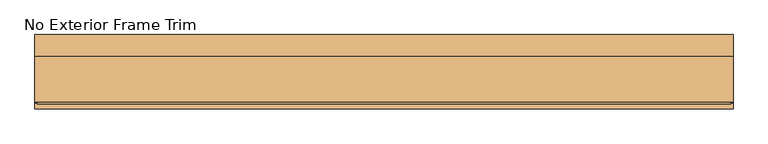
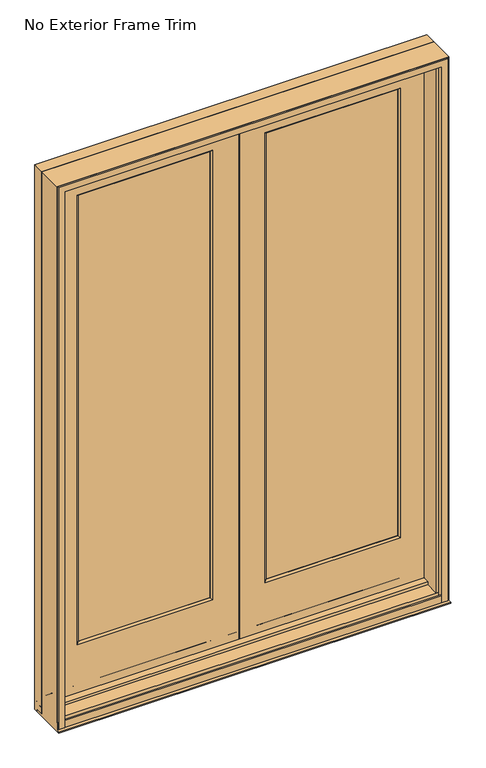
"""IFC4 building model written with IfcOpenShell, lengths in millimetres: door geometry, Door-In_Swing-Milgard-Essence-2_Panel : No Exterior Frame Trim."""

from ifc_helpers import new_model, si_unit, frame, origin, place, context, project, spatial, polyline, outline, extrude, faceted_brep, source, transform, mapped, element, save


def no_exterior_frame_trim_898b5155(model_context):
    return source(origin(), model_context, "Body", "SolidModel", [
        extrude(outline(polyline([(591.4684989, -34.925), (54.2422052, -34.925), (54.2422052, -9.525), (591.4684989, -9.525), (591.4684989, -34.925)])), frame((0.0, 0.0, 245.0465023), z_axis=(0.0, 0.0, 1.0), x_axis=(1.0, 0.0, 0.0)), (0.0, 0.0, 1.0), 1856.965426),
        faceted_brep([(-22.501829, -7.1755004, 39.0524923), (-39.8139839, -7.1755004, 39.0524923), (-39.8139839, 1.1430002, 39.0524923), (685.524688, 1.1430002, 39.0524923), (685.524688, -7.1755004, 39.0524923), (668.2125331, -7.1755004, 39.0524923), (665.7443122, -10.2234994, 39.0524923), (597.9581931, -10.2234994, 39.0524923), (597.9581931, -8.4581998, 39.0524923), (583.7647037, -8.4581998, 39.0524923), (582.2411552, -9.525, 39.0524923), (578.7581009, -9.525, 39.0524923), (578.7581009, -7.642861, 39.0524923), (579.0279319, -7.1755004, 39.0524923), (66.6827722, -7.1755004, 39.0524923), (66.9526032, -7.642861, 39.0524923), (66.9526032, -9.525, 39.0524923), (63.4695489, -9.525, 39.0524923), (61.9460004, -8.4581998, 39.0524923), (47.7525111, -8.4581998, 39.0524923), (47.7525111, -10.2234994, 39.0524923), (-20.0336081, -10.2234994, 39.0524923), (-22.501829, -7.1755004, 2178.7559624), (-22.501829, -7.1755004, 257.4235308), (-22.1233678, -7.642861, 257.6933617), (-20.5992417, -9.525, 257.6933617), (-20.5992417, -9.525, 254.2103075), (-21.4631194, -8.4581998, 252.686759), (-21.4631194, -8.4581998, 238.4932696), (-20.0336081, -10.2234994, 238.4932696), (-20.0336081, -10.2234994, 2176.2877415), (-20.0336081, -10.2234994, 58.8285873), (-22.501829, -7.1755004, 56.3603664), (47.7525111, -10.2234994, 58.8285873), (597.9581931, -10.2234994, 58.8285873), (665.7443122, -10.2234994, 58.8285873), (685.524688, -10.2234994, 58.8285873), (685.524688, -10.2234994, 238.4932696), (665.7443122, -10.2234994, 238.4932696), (665.7443122, -10.2234994, 2176.2877415), (-39.8139839, -10.2234994, 238.4932696), (-39.8139839, -10.2234994, 58.8285873), (47.7525111, -10.2234994, 2108.5016224), (597.9581931, -10.2234994, 2108.5016224), (597.9581931, -10.2234994, 238.4932696), (47.7525111, -10.2234994, 238.4932696), (47.7525111, -8.4581998, 238.4932696), (47.7525111, -8.4581998, 252.686759), (47.7525111, -9.525, 254.2103075), (47.7525111, -9.525, 257.6933617), (47.7525111, -8.4581998, 257.6933617), (47.7525111, -8.4581998, 2108.5016224), (47.7525111, -8.4581998, 57.3990759), (597.9581931, -8.4581998, 57.3990759), (583.7647037, -8.4581998, 57.3990759), (61.9460004, -8.4581998, 238.4932696), (61.9460004, -8.4581998, 252.686759), (61.9460004, -8.4581998, 257.6933617), (61.9460004, -8.4581998, 2094.3081331), (583.7647037, -8.4581998, 2094.3081331), (583.7647037, -8.4581998, 257.6933617), (597.9581931, -8.4581998, 257.6933617), (597.9581931, -8.4581998, 2108.5016224), (597.9581931, -8.4581998, 252.686759), (583.7647037, -8.4581998, 252.686759), (583.7647037, -8.4581998, 238.4932696), (597.9581931, -8.4581998, 238.4932696), (61.9460004, -8.4581998, 57.3990759), (63.4695489, -9.525, 238.4932696), (63.4695489, -9.525, 254.2103075), (63.4695489, -9.525, 257.6933617), (63.4695489, -9.525, 2092.7845845), (63.4695489, -9.525, 58.2629537), (582.2411552, -9.525, 58.2629537), (578.7581009, -9.525, 58.2629537), (66.9526032, -9.525, 238.4932696), (66.9526032, -9.525, 254.2103075), (578.7581009, -9.525, 254.2103075), (578.7581009, -9.525, 238.4932696), (582.2411552, -9.525, 238.4932696), (582.2411552, -9.525, 254.2103075), (597.9581931, -9.525, 254.2103075), (597.9581931, -9.525, 257.6933617), (582.2411552, -9.525, 257.6933617), (582.2411552, -9.525, 2092.7845845), (66.9526032, -9.525, 2089.3015303), (578.7581009, -9.525, 2089.3015303), (578.7581009, -9.525, 257.6933617), (66.9526032, -9.525, 257.6933617), (685.524688, -9.525, 257.6933617), (666.3099458, -9.525, 257.6933617), (666.3099458, -9.525, 254.2103075), (685.524688, -9.525, 254.2103075), (66.9526032, -9.525, 58.2629537), (-39.8139839, -9.525, 254.2103075), (-39.8139839, -9.525, 257.6933617), (66.9526032, -8.4581998, 238.4932696), (66.9526032, -8.4581998, 252.686759), (66.9526032, -7.642861, 257.6933617), (66.9526032, -7.642861, 2089.3015303), (66.9526032, -7.642861, 56.7388275), (66.6827722, -7.1755004, 56.3603664), (62.3383529, 0.3492502, 253.0791115), (62.3383529, 0.3492502, 2093.9157805), (597.9581931, 0.3492502, 2108.5016224), (597.9581931, 0.3492502, 238.4932696), (47.7525111, 0.3492502, 238.4932696), (47.7525111, 0.3492502, 2108.5016224), (583.3723512, 0.3492502, 253.0791115), (583.3723512, 0.3492502, 2093.9157805), (47.7525111, 1.1430002, 238.4932696), (47.7525111, 1.1430002, 2108.5016224), (-39.8139839, 1.1430002, 2196.0681173), (685.524688, 1.1430002, 2196.0681173), (597.9581931, 1.1430002, 2108.5016224), (597.9581931, 1.1430002, 238.4932696), (-39.8139839, -7.1755004, 56.3603664), (-39.8139839, -8.4581998, 238.4932696), (-39.8139839, -8.4581998, 252.686759), (-39.8139839, -7.642861, 257.6933617), (-39.8139839, -7.1755004, 257.4235308), (-39.8139839, -7.1755004, 2196.0681173), (685.524688, -7.1755004, 56.3603664), (668.2125331, -7.1755004, 56.3603664), (668.2125331, -7.1755004, 2178.7559624), (668.2125331, -7.1755004, 257.4235308), (685.524688, -7.1755004, 257.4235308), (685.524688, -7.1755004, 2196.0681173), (578.7581009, -7.642861, 2089.3015303), (667.1738236, -8.4581998, 238.4932696), (667.1738236, -8.4581998, 252.686759), (667.8340719, -7.642861, 257.6933617), (578.7581009, -7.642861, 56.7388275), (578.7581009, -8.4581998, 252.686759), (578.7581009, -8.4581998, 238.4932696), (578.7581009, -7.642861, 257.6933617), (579.0279319, -7.1755004, 56.3603664), (685.524688, -7.642861, 257.6933617), (685.524688, -8.4581998, 252.686759), (685.524688, -8.4581998, 238.4932696)], [[[0, 1, 2, 3, 4, 5, 6, 7, 8, 9, 10, 11, 12, 13, 14, 15, 16, 17, 18, 19, 20, 21]], [[22, 23, 24, 25, 26, 27, 28, 29, 30]], [[21, 31, 32, 0]], [[20, 33, 34, 7, 6, 35, 36, 37, 38, 39, 30, 29, 40, 41, 31, 21], [42, 43, 44, 45]], [[42, 45, 46, 47, 48, 49, 50, 51]], [[19, 52, 33, 20]], [[8, 53, 54, 9]], [[46, 55, 56, 47]], [[51, 50, 57, 58, 59, 60, 61, 62]], [[63, 64, 65, 66]], [[18, 67, 52, 19]], [[55, 68, 69, 56]], [[58, 57, 70, 71]], [[17, 72, 67, 18]], [[10, 73, 74, 11]], [[71, 70, 49, 48, 69, 68, 75, 76, 77, 78, 79, 80, 81, 82, 83, 84], [85, 86, 87, 88]], [[89, 90, 91, 92]], [[16, 93, 72, 17]], [[94, 26, 25, 95]], [[75, 96, 97, 76]], [[85, 88, 98, 99]], [[15, 100, 93, 16]], [[14, 101, 100, 15]], [[99, 98, 102, 103]], [[104, 105, 106, 107], [103, 102, 108, 109]], [[106, 110, 111, 107]], [[2, 112, 113, 3], [114, 111, 110, 115]], [[1, 116, 41, 40, 117, 118, 94, 95, 119, 120, 121, 112, 2]], [[0, 32, 116, 1]], [[4, 122, 123, 5]], [[121, 120, 23, 22, 124, 125, 126, 127]], [[30, 39, 124, 22]], [[42, 51, 62, 43]], [[58, 71, 84, 59]], [[85, 99, 128, 86]], [[103, 109, 128, 99]], [[107, 111, 114, 104]], [[112, 121, 127, 113]], [[39, 38, 129, 130, 91, 90, 131, 125, 124]], [[5, 123, 35, 6]], [[62, 61, 82, 81, 63, 66, 44, 43]], [[7, 34, 53, 8]], [[84, 83, 60, 59]], [[9, 54, 73, 10]], [[79, 65, 64, 80]], [[11, 74, 132, 12]], [[77, 133, 134, 78]], [[128, 135, 87, 86]], [[109, 108, 135, 128]], [[12, 132, 136, 13]], [[114, 115, 105, 104]], [[127, 126, 137, 89, 92, 138, 139, 37, 36, 122, 4, 3, 113]], [[105, 115, 110, 106]], [[102, 98, 135, 108]], [[126, 125, 131, 137]], [[119, 24, 23, 120]], [[70, 57, 50, 49]], [[95, 25, 24, 119]], [[82, 61, 60, 83]], [[87, 135, 98, 88]], [[137, 131, 90, 89]], [[48, 47, 56, 69]], [[76, 97, 133, 77]], [[80, 64, 63, 81]], [[92, 91, 130, 138]], [[118, 27, 26, 94]], [[97, 96, 134, 133]], [[138, 130, 129, 139]], [[117, 28, 27, 118]], [[40, 29, 28, 117]], [[44, 66, 65, 79, 78, 134, 96, 75, 68, 55, 46, 45]], [[139, 129, 38, 37]], [[33, 52, 67, 72, 93, 100, 101, 136, 132, 74, 73, 54, 53, 34]], [[116, 32, 31, 41]], [[36, 35, 123, 122]], [[13, 136, 101, 14]]]),
        faceted_brep([(-39.8139839, -43.3070016, 39.0524923), (-39.8139839, -43.3070016, 2196.0681173), (-39.8139839, -7.1755004, 2196.0681173), (-39.8139839, -7.1755004, 39.0524923), (685.524688, -7.1755004, 39.0524923), (685.524688, -7.1755004, 2196.0681173), (685.524688, -43.3070016, 2196.0681173), (685.524688, -43.3070016, 39.0524923), (66.7863819, -36.1729967, 257.5271404), (59.6523769, -43.3070016, 250.3931355), (586.0583272, -43.3070016, 250.3931355), (578.9243222, -36.1729967, 257.5271404), (59.6523769, -43.3070016, 2096.6017565), (586.0583272, -43.3070016, 2096.6017565), (669.6356705, -7.1755004, 55.4786786), (669.6356705, -7.1755004, 2180.1790999), (-23.9249664, -7.1755004, 2180.1790999), (-23.9249664, -7.1755004, 55.4786786), (-20.8769674, -10.2234994, 57.9468995), (666.5876715, -10.2234994, 57.9468995), (666.5876715, -10.2234994, 2177.1311009), (-20.8769674, -10.2234994, 2177.1311009), (594.7531877, -10.2234994, 241.698275), (594.7531877, -10.2234994, 2105.296617), (50.9575164, -10.2234994, 2105.296617), (50.9575164, -10.2234994, 241.698275), (50.9575164, -12.6518919, 241.698275), (594.7531877, -12.6518919, 241.698275), (49.0643221, -12.6518919, 2107.1898114), (49.0643221, -12.6518919, 239.8050807), (596.646382, -12.6518919, 239.8050807), (596.646382, -12.6518919, 2107.1898114), (50.9575164, -12.6518919, 2105.296617), (594.7531877, -12.6518919, 2105.296617), (47.7525111, -16.6892311, 238.4932696), (597.9581931, -16.6892311, 238.4932696), (47.7525111, -35.6615995, 238.4932696), (64.012343, -35.6615995, 238.4932696), (64.7489425, -34.925, 238.4932696), (66.7863819, -34.925, 238.4932696), (66.7863819, -35.6615995, 238.4932696), (578.9243222, -35.6615995, 238.4932696), (578.9243222, -34.925, 238.4932696), (580.9617616, -34.925, 238.4932696), (581.6983611, -35.6615995, 238.4932696), (597.9581931, -35.6615995, 238.4932696), (581.6983611, -35.6615995, 254.7531016), (597.9581931, -35.6615995, 254.7531016), (66.7863819, -35.6615995, 254.7531016), (578.9243222, -35.6615995, 254.7531016), (47.7525111, -35.6615995, 254.7531016), (64.012343, -35.6615995, 254.7531016), (47.7525111, -34.925, 255.4897011), (64.7489425, -34.925, 255.4897011), (66.7863819, -34.925, 255.4897011), (578.9243222, -34.925, 255.4897011), (580.9617616, -34.925, 255.4897011), (597.9581931, -34.925, 255.4897011), (47.7525111, -34.925, 257.5271404), (64.7489425, -34.925, 257.5271404), (64.7489425, -34.925, 2091.505191), (580.9617616, -34.925, 2091.505191), (580.9617616, -34.925, 257.5271404), (597.9581931, -34.925, 257.5271404), (578.9243222, -34.925, 257.5271404), (578.9243222, -34.925, 2089.4677516), (66.7863819, -34.925, 2089.4677516), (66.7863819, -34.925, 257.5271404), (581.6983611, -35.6615995, 257.5271404), (597.9581931, -35.6615995, 257.5271404), (47.7525111, -35.6615995, 257.5271404), (64.012343, -35.6615995, 257.5271404), (66.7863819, -36.1729967, 2089.4677516), (64.012343, -35.6615995, 2092.2417904), (47.7525111, -35.6615995, 2108.5016224), (597.9581931, -35.6615995, 2108.5016224), (581.6983611, -35.6615995, 2092.2417904), (47.7525111, -16.6892311, 2108.5016224), (578.9243222, -36.1729967, 2089.4677516), (597.9581931, -16.6892311, 2108.5016224)], [[[0, 1, 2, 3]], [[4, 5, 6, 7]], [[8, 9, 10, 11]], [[0, 7, 6, 1], [9, 12, 13, 10]], [[4, 7, 0, 3]], [[2, 5, 4, 3], [14, 15, 16, 17]], [[17, 18, 19, 14]], [[20, 19, 18, 21], [22, 23, 24, 25]], [[25, 26, 27, 22]], [[28, 29, 30, 31], [26, 32, 33, 27]], [[29, 34, 35, 30]], [[34, 36, 37, 38, 39, 40, 41, 42, 43, 44, 45, 35]], [[44, 46, 47, 45]], [[40, 48, 49, 41]], [[36, 50, 51, 37]], [[50, 52, 53, 51]], [[48, 54, 55, 49]], [[46, 56, 57, 47]], [[52, 58, 59, 60, 61, 62, 63, 57, 56, 43, 42, 55, 54, 39, 38, 53], [64, 65, 66, 67]], [[11, 64, 67, 8]], [[62, 68, 69, 63]], [[58, 70, 71, 59]], [[12, 9, 8, 72]], [[54, 48, 40, 39]], [[72, 8, 67, 66]], [[38, 37, 51, 53]], [[60, 59, 71, 73]], [[73, 71, 70, 74, 75, 69, 68, 76]], [[74, 70, 58, 52, 50, 36, 34, 77]], [[77, 34, 29, 28]], [[32, 26, 25, 24]], [[18, 17, 16, 21]], [[12, 72, 78, 13]], [[66, 65, 78, 72]], [[60, 73, 76, 61]], [[74, 77, 79, 75]], [[28, 31, 79, 77]], [[32, 24, 23, 33]], [[21, 16, 15, 20]], [[6, 5, 2, 1]], [[78, 11, 10, 13]], [[42, 41, 49, 55]], [[65, 64, 11, 78]], [[56, 46, 44, 43]], [[76, 68, 62, 61]], [[79, 35, 45, 47, 57, 63, 69, 75]], [[30, 35, 79, 31]], [[23, 22, 27, 33]], [[15, 14, 19, 20]]]),
        extrude(outline(polyline([(-675.754549, -34.925), (-675.754549, -9.525), (-138.5282552, -9.525), (-138.5282552, -34.925), (-675.754549, -34.925)])), frame((0.0, 0.0, 245.0465023), z_axis=(0.0, 0.0, 1.0), x_axis=(1.0, 0.0, 0.0)), (0.0, 0.0, 1.0), 1856.965426),
        faceted_brep([(-61.784221, -7.1755004, 39.0524923), (-64.252442, -10.2234994, 39.0524923), (-132.0385611, -10.2234994, 39.0524923), (-132.0385611, -8.4581998, 39.0524923), (-146.2320504, -8.4581998, 39.0524923), (-147.755599, -9.525, 39.0524923), (-151.2386532, -9.525, 39.0524923), (-151.2386532, -7.642861, 39.0524923), (-150.9688223, -7.1755004, 39.0524923), (-663.3139819, -7.1755004, 39.0524923), (-663.044151, -7.642861, 39.0524923), (-663.044151, -9.525, 39.0524923), (-666.5272052, -9.525, 39.0524923), (-668.0507537, -8.4581998, 39.0524923), (-682.2442431, -8.4581998, 39.0524923), (-682.2442431, -10.2234994, 39.0524923), (-750.0303622, -10.2234994, 39.0524923), (-752.4985831, -7.1755004, 39.0524923), (-769.810738, -7.1755004, 39.0524923), (-769.810738, 1.1430002, 39.0524923), (-44.4720661, 1.1430002, 39.0524923), (-44.4720661, -7.1755004, 39.0524923), (-61.784221, -7.1755004, 56.3603664), (-64.252442, -10.2234994, 58.8285873), (-61.784221, -7.1755004, 2178.7559624), (-64.252442, -10.2234994, 2176.2877415), (-64.252442, -10.2234994, 238.4932696), (-62.8229306, -8.4581998, 238.4932696), (-62.8229306, -8.4581998, 252.686759), (-63.6868083, -9.525, 254.2103075), (-63.6868083, -9.525, 257.6933617), (-62.1626822, -7.642861, 257.6933617), (-61.784221, -7.1755004, 257.4235308), (-44.4720661, -10.2234994, 58.8285873), (-44.4720661, -10.2234994, 238.4932696), (-750.0303622, -10.2234994, 2176.2877415), (-750.0303622, -10.2234994, 238.4932696), (-769.810738, -10.2234994, 238.4932696), (-769.810738, -10.2234994, 58.8285873), (-750.0303622, -10.2234994, 58.8285873), (-682.2442431, -10.2234994, 58.8285873), (-132.0385611, -10.2234994, 58.8285873), (-132.0385611, -10.2234994, 2108.5016224), (-132.0385611, -10.2234994, 238.4932696), (-682.2442431, -10.2234994, 238.4932696), (-682.2442431, -10.2234994, 2108.5016224), (-132.0385611, -8.4581998, 57.3990759), (-132.0385611, -8.4581998, 2108.5016224), (-132.0385611, -8.4581998, 257.6933617), (-132.0385611, -9.525, 257.6933617), (-132.0385611, -9.525, 254.2103075), (-132.0385611, -8.4581998, 252.686759), (-132.0385611, -8.4581998, 238.4932696), (-668.0507537, -8.4581998, 57.3990759), (-682.2442431, -8.4581998, 57.3990759), (-146.2320504, -8.4581998, 57.3990759), (-682.2442431, -8.4581998, 2108.5016224), (-682.2442431, -8.4581998, 257.6933617), (-668.0507537, -8.4581998, 257.6933617), (-668.0507537, -8.4581998, 2094.3081331), (-146.2320504, -8.4581998, 2094.3081331), (-146.2320504, -8.4581998, 257.6933617), (-146.2320504, -8.4581998, 252.686759), (-146.2320504, -8.4581998, 238.4932696), (-682.2442431, -8.4581998, 252.686759), (-682.2442431, -8.4581998, 238.4932696), (-668.0507537, -8.4581998, 238.4932696), (-668.0507537, -8.4581998, 252.686759), (-147.755599, -9.525, 58.2629537), (-147.755599, -9.525, 2092.7845845), (-147.755599, -9.525, 257.6933617), (-147.755599, -9.525, 254.2103075), (-147.755599, -9.525, 238.4932696), (-663.044151, -9.525, 58.2629537), (-666.5272052, -9.525, 58.2629537), (-151.2386532, -9.525, 58.2629537), (-666.5272052, -9.525, 2092.7845845), (-666.5272052, -9.525, 257.6933617), (-682.2442431, -9.525, 257.6933617), (-682.2442431, -9.525, 254.2103075), (-666.5272052, -9.525, 254.2103075), (-666.5272052, -9.525, 238.4932696), (-663.044151, -9.525, 238.4932696), (-663.044151, -9.525, 254.2103075), (-151.2386532, -9.525, 254.2103075), (-151.2386532, -9.525, 238.4932696), (-151.2386532, -9.525, 2089.3015303), (-151.2386532, -9.525, 257.6933617), (-663.044151, -9.525, 257.6933617), (-663.044151, -9.525, 2089.3015303), (-44.4720661, -9.525, 254.2103075), (-44.4720661, -9.525, 257.6933617), (-769.810738, -9.525, 257.6933617), (-769.810738, -9.525, 254.2103075), (-750.5959958, -9.525, 254.2103075), (-750.5959958, -9.525, 257.6933617), (-151.2386532, -7.642861, 56.7388275), (-151.2386532, -7.642861, 2089.3015303), (-151.2386532, -7.642861, 257.6933617), (-151.2386532, -8.4581998, 252.686759), (-151.2386532, -8.4581998, 238.4932696), (-150.9688223, -7.1755004, 56.3603664), (-146.624403, 0.3492502, 2093.9157805), (-146.624403, 0.3492502, 253.0791115), (-682.2442431, 0.3492502, 2108.5016224), (-132.0385611, 0.3492502, 2108.5016224), (-132.0385611, 0.3492502, 238.4932696), (-682.2442431, 0.3492502, 238.4932696), (-667.6584012, 0.3492502, 2093.9157805), (-667.6584012, 0.3492502, 253.0791115), (-132.0385611, 1.1430002, 2108.5016224), (-132.0385611, 1.1430002, 238.4932696), (-769.810738, 1.1430002, 2196.0681173), (-44.4720661, 1.1430002, 2196.0681173), (-682.2442431, 1.1430002, 2108.5016224), (-682.2442431, 1.1430002, 238.4932696), (-44.4720661, -7.1755004, 2196.0681173), (-44.4720661, -7.1755004, 257.4235308), (-44.4720661, -7.642861, 257.6933617), (-44.4720661, -8.4581998, 252.686759), (-44.4720661, -8.4581998, 238.4932696), (-44.4720661, -7.1755004, 56.3603664), (-752.4985831, -7.1755004, 56.3603664), (-769.810738, -7.1755004, 56.3603664), (-769.810738, -7.1755004, 2196.0681173), (-769.810738, -7.1755004, 257.4235308), (-752.4985831, -7.1755004, 257.4235308), (-752.4985831, -7.1755004, 2178.7559624), (-663.044151, -7.642861, 2089.3015303), (-752.120122, -7.642861, 257.6933617), (-751.4598736, -8.4581998, 252.686759), (-751.4598736, -8.4581998, 238.4932696), (-663.044151, -7.642861, 56.7388275), (-663.044151, -7.642861, 257.6933617), (-663.044151, -8.4581998, 238.4932696), (-663.044151, -8.4581998, 252.686759), (-663.3139819, -7.1755004, 56.3603664), (-769.810738, -8.4581998, 238.4932696), (-769.810738, -8.4581998, 252.686759), (-769.810738, -7.642861, 257.6933617)], [[[0, 1, 2, 3, 4, 5, 6, 7, 8, 9, 10, 11, 12, 13, 14, 15, 16, 17, 18, 19, 20, 21]], [[1, 0, 22, 23]], [[24, 25, 26, 27, 28, 29, 30, 31, 32]], [[2, 1, 23, 33, 34, 26, 25, 35, 36, 37, 38, 39, 16, 15, 40, 41], [42, 43, 44, 45]], [[3, 2, 41, 46]], [[42, 47, 48, 49, 50, 51, 52, 43]], [[14, 13, 53, 54]], [[4, 3, 46, 55]], [[47, 56, 57, 58, 59, 60, 61, 48]], [[52, 51, 62, 63]], [[64, 65, 66, 67]], [[5, 4, 55, 68]], [[60, 69, 70, 61]], [[63, 62, 71, 72]], [[12, 11, 73, 74]], [[6, 5, 68, 75]], [[69, 76, 77, 78, 79, 80, 81, 82, 83, 84, 85, 72, 71, 50, 49, 70], [86, 87, 88, 89]], [[90, 91, 30, 29]], [[92, 93, 94, 95]], [[7, 6, 75, 96]], [[86, 97, 98, 87]], [[85, 84, 99, 100]], [[8, 7, 96, 101]], [[97, 102, 103, 98]], [[104, 105, 106, 107], [102, 108, 109, 103]], [[106, 105, 110, 111]], [[20, 19, 112, 113], [114, 115, 111, 110]], [[21, 20, 113, 116, 117, 118, 91, 90, 119, 120, 34, 33, 121]], [[0, 21, 121, 22]], [[18, 17, 122, 123]], [[116, 124, 125, 126, 127, 24, 32, 117]], [[25, 24, 127, 35]], [[42, 45, 56, 47]], [[60, 59, 76, 69]], [[86, 89, 128, 97]], [[102, 97, 128, 108]], [[105, 104, 114, 110]], [[113, 112, 124, 116]], [[17, 16, 39, 122]], [[35, 127, 126, 129, 95, 94, 130, 131, 36]], [[15, 14, 54, 40]], [[56, 45, 44, 65, 64, 79, 78, 57]], [[13, 12, 74, 53]], [[81, 80, 67, 66]], [[76, 59, 58, 77]], [[11, 10, 132, 73]], [[128, 89, 88, 133]], [[83, 82, 134, 135]], [[10, 9, 136, 132]], [[108, 128, 133, 109]], [[114, 104, 107, 115]], [[124, 112, 19, 18, 123, 38, 37, 137, 138, 93, 92, 139, 125]], [[107, 106, 111, 115]], [[118, 117, 32, 31]], [[125, 139, 129, 126]], [[103, 109, 133, 98]], [[70, 49, 48, 61]], [[78, 77, 58, 57]], [[88, 87, 98, 133]], [[91, 118, 31, 30]], [[139, 92, 95, 129]], [[119, 90, 29, 28]], [[93, 138, 130, 94]], [[50, 71, 62, 51]], [[84, 83, 135, 99]], [[80, 79, 64, 67]], [[120, 119, 28, 27]], [[138, 137, 131, 130]], [[99, 135, 134, 100]], [[44, 43, 52, 63, 72, 85, 100, 134, 82, 81, 66, 65]], [[34, 120, 27, 26]], [[137, 37, 36, 131]], [[121, 33, 23, 22]], [[38, 123, 122, 39]], [[41, 40, 54, 53, 74, 73, 132, 136, 101, 96, 75, 68, 55, 46]], [[9, 8, 101, 136]]]),
        faceted_brep([(-44.4720661, -43.3070016, 39.0524923), (-44.4720661, -7.1755004, 39.0524923), (-44.4720661, -7.1755004, 2196.0681173), (-44.4720661, -43.3070016, 2196.0681173), (-769.810738, -7.1755004, 39.0524923), (-769.810738, -43.3070016, 39.0524923), (-769.810738, -43.3070016, 2196.0681173), (-769.810738, -7.1755004, 2196.0681173), (-151.0724319, -36.1729967, 257.5271404), (-663.2103723, -36.1729967, 257.5271404), (-670.3443772, -43.3070016, 250.3931355), (-143.938427, -43.3070016, 250.3931355), (-670.3443772, -43.3070016, 2096.6017565), (-143.938427, -43.3070016, 2096.6017565), (-753.9217206, -7.1755004, 55.4786786), (-60.3610836, -7.1755004, 55.4786786), (-60.3610836, -7.1755004, 2180.1790999), (-753.9217206, -7.1755004, 2180.1790999), (-750.8737216, -10.2234994, 57.9468995), (-63.4090826, -10.2234994, 57.9468995), (-750.8737216, -10.2234994, 2177.1311009), (-63.4090826, -10.2234994, 2177.1311009), (-679.0392377, -10.2234994, 241.698275), (-135.2435664, -10.2234994, 241.698275), (-135.2435664, -10.2234994, 2105.296617), (-679.0392377, -10.2234994, 2105.296617), (-679.0392377, -12.6518919, 241.698275), (-135.2435664, -12.6518919, 241.698275), (-133.3503721, -12.6518919, 2107.1898114), (-680.9324321, -12.6518919, 2107.1898114), (-680.9324321, -12.6518919, 239.8050807), (-133.3503721, -12.6518919, 239.8050807), (-679.0392377, -12.6518919, 2105.296617), (-135.2435664, -12.6518919, 2105.296617), (-682.2442431, -16.6892311, 238.4932696), (-132.0385611, -16.6892311, 238.4932696), (-682.2442431, -35.6615995, 238.4932696), (-665.9844111, -35.6615995, 238.4932696), (-665.2478116, -34.925, 238.4932696), (-663.2103723, -34.925, 238.4932696), (-663.2103723, -35.6615995, 238.4932696), (-151.0724319, -35.6615995, 238.4932696), (-151.0724319, -34.925, 238.4932696), (-149.0349925, -34.925, 238.4932696), (-148.298393, -35.6615995, 238.4932696), (-132.0385611, -35.6615995, 238.4932696), (-148.298393, -35.6615995, 254.7531016), (-132.0385611, -35.6615995, 254.7531016), (-663.2103723, -35.6615995, 254.7531016), (-151.0724319, -35.6615995, 254.7531016), (-682.2442431, -35.6615995, 254.7531016), (-665.9844111, -35.6615995, 254.7531016), (-149.0349925, -34.925, 255.4897011), (-132.0385611, -34.925, 255.4897011), (-663.2103723, -34.925, 255.4897011), (-151.0724319, -34.925, 255.4897011), (-682.2442431, -34.925, 255.4897011), (-665.2478116, -34.925, 255.4897011), (-682.2442431, -34.925, 257.5271404), (-665.2478116, -34.925, 257.5271404), (-665.2478116, -34.925, 2091.505191), (-149.0349925, -34.925, 2091.505191), (-149.0349925, -34.925, 257.5271404), (-132.0385611, -34.925, 257.5271404), (-663.2103723, -34.925, 257.5271404), (-151.0724319, -34.925, 257.5271404), (-151.0724319, -34.925, 2089.4677516), (-663.2103723, -34.925, 2089.4677516), (-148.298393, -35.6615995, 257.5271404), (-132.0385611, -35.6615995, 257.5271404), (-682.2442431, -35.6615995, 257.5271404), (-665.9844111, -35.6615995, 257.5271404), (-151.0724319, -36.1729967, 2089.4677516), (-148.298393, -35.6615995, 2092.2417904), (-665.9844111, -35.6615995, 2092.2417904), (-682.2442431, -35.6615995, 2108.5016224), (-132.0385611, -35.6615995, 2108.5016224), (-132.0385611, -16.6892311, 2108.5016224), (-663.2103723, -36.1729967, 2089.4677516), (-682.2442431, -16.6892311, 2108.5016224)], [[[0, 1, 2, 3]], [[4, 5, 6, 7]], [[8, 9, 10, 11]], [[0, 3, 6, 5], [11, 10, 12, 13]], [[4, 1, 0, 5]], [[2, 1, 4, 7], [14, 15, 16, 17]], [[15, 14, 18, 19]], [[20, 21, 19, 18], [22, 23, 24, 25]], [[23, 22, 26, 27]], [[28, 29, 30, 31], [27, 26, 32, 33]], [[31, 30, 34, 35]], [[35, 34, 36, 37, 38, 39, 40, 41, 42, 43, 44, 45]], [[45, 44, 46, 47]], [[41, 40, 48, 49]], [[37, 36, 50, 51]], [[47, 46, 52, 53]], [[49, 48, 54, 55]], [[51, 50, 56, 57]], [[53, 52, 43, 42, 55, 54, 39, 38, 57, 56, 58, 59, 60, 61, 62, 63], [64, 65, 66, 67]], [[9, 8, 65, 64]], [[63, 62, 68, 69]], [[59, 58, 70, 71]], [[13, 72, 8, 11]], [[55, 42, 41, 49]], [[72, 66, 65, 8]], [[43, 52, 46, 44]], [[61, 73, 68, 62]], [[73, 74, 71, 70, 75, 76, 69, 68]], [[76, 77, 35, 45, 47, 53, 63, 69]], [[77, 28, 31, 35]], [[33, 24, 23, 27]], [[19, 21, 16, 15]], [[13, 12, 78, 72]], [[66, 72, 78, 67]], [[61, 60, 74, 73]], [[76, 75, 79, 77]], [[28, 77, 79, 29]], [[33, 32, 25, 24]], [[21, 20, 17, 16]], [[6, 3, 2, 7]], [[78, 12, 10, 9]], [[39, 54, 48, 40]], [[67, 78, 9, 64]], [[74, 60, 59, 71]], [[57, 38, 37, 51]], [[79, 75, 70, 58, 56, 50, 36, 34]], [[30, 29, 79, 34]], [[25, 32, 26, 22]], [[17, 20, 18, 14]]]),
        faceted_brep([(719.8791802, 11.1125, 0.0), (719.8791802, 11.1125, 2235.2), (719.8791802, -35.8012989, 2235.2), (719.8791802, -35.7981518, 9.128125), (719.8791802, -1.5874989, 9.128125), (719.8791802, -1.5874989, 0.0), (-804.1208198, -1.5874989, 0.0), (-804.1208198, -1.5874989, 9.128125), (-804.1208198, -35.7981518, 9.128125), (-804.1208198, -35.8012989, 2235.2), (-804.1208198, 11.1125, 2235.2), (-804.1208198, 11.1125, 0.0), (-775.5465905, 11.1125, 41.6602461), (691.3049508, 11.1125, 41.6602461), (691.3049508, 11.1125, 2206.6257706), (-775.5465905, 11.1125, 2206.6257706), (688.7641767, -1.5874989, 9.128125), (688.7641767, -1.5874989, 40.5405728), (-773.0058163, -1.5874989, 40.5405728), (-773.0058163, -1.5874989, 9.128125), (693.7179256, -35.7981518, 9.128125), (693.7179256, -13.2714994, 9.128125), (691.304169, -13.2714994, 9.128125), (691.304169, -8.47231, 9.128125), (688.7641767, -8.47231, 9.128125), (-777.9595653, -35.7981518, 9.128125), (-773.0058163, -8.47231, 9.128125), (-775.5458087, -8.47231, 9.128125), (-775.5458087, -13.2714994, 9.128125), (-777.9595653, -13.2714994, 9.128125), (688.7641767, 2.7127992, 41.2988289), (691.3049508, 2.7127992, 41.2988289), (691.3049508, 4.7625043, 41.6602461), (-775.5465905, 4.7625043, 41.6602461), (-775.5465905, 2.7127992, 41.2988289), (-773.0058163, 2.7127992, 41.2988289), (691.3049508, 2.7127992, 2206.6257706), (688.7641767, 2.7127992, 2204.0849965), (-773.0058163, 2.7127992, 2204.0849965), (-775.5465905, 2.7127992, 2206.6257706), (688.7641767, -8.47231, 2204.0849965), (-773.0058163, -8.47231, 2204.0849965), (691.304169, -8.47231, 2206.6249888), (-775.5458087, -8.47231, 2206.6249888), (-777.9595653, -35.8012989, 2209.0380233), (-777.9595653, -13.2714994, 2209.0380233), (693.7179256, -13.2714994, 2209.0380233), (693.7179256, -35.8012989, 2209.0380233), (691.304169, -13.2714994, 2206.6249888), (-775.5458087, -13.2714994, 2206.6249888)], [[[0, 1, 2, 3, 4, 5]], [[6, 7, 8, 9, 10, 11]], [[10, 1, 0, 11], [12, 13, 14, 15]], [[5, 4, 16, 17, 18, 19, 7, 6]], [[5, 6, 11, 0]], [[20, 21, 22, 23, 24, 16, 4, 3]], [[25, 8, 7, 19, 26, 27, 28, 29]], [[17, 30, 31, 32, 33, 34, 35, 18]], [[12, 33, 32, 13]], [[36, 31, 30, 37, 38, 35, 34, 39]], [[37, 40, 41, 38]], [[40, 24, 23, 42, 43, 27, 26, 41]], [[44, 45, 46, 47]], [[2, 9, 8, 25, 44, 47, 20, 3]], [[1, 10, 9, 2]], [[39, 15, 14, 36]], [[13, 32, 31, 36, 14]], [[40, 37, 30, 17, 16, 24]], [[22, 48, 42, 23]], [[21, 46, 45, 29, 28, 49, 48, 22]], [[20, 47, 46, 21]], [[48, 49, 43, 42]], [[15, 39, 34, 33, 12]], [[26, 19, 18, 35, 38, 41]], [[43, 49, 28, 27]], [[29, 45, 44, 25]]]),
        faceted_brep([(719.8791802, -150.7170398, 0.0007738), (719.8791802, -1.5874989, 0.0007738), (719.8791802, -1.5874989, 40.9473783), (719.8791802, -7.9374984, 39.2302591), (719.8791802, -7.9374984, 36.0475021), (719.8791802, -35.7981518, 34.0993068), (719.8791802, -35.7981518, 2235.2), (719.8791802, -135.8899958, 2235.2), (719.8791802, -135.8899958, 33.0268847), (719.8791802, -138.0870975, 32.7181022), (719.8791802, -138.0870975, 4.9752253), (719.8791802, -150.7170398, 3.8703788), (-804.1208198, -1.5874989, 0.0007738), (-804.1208198, -150.7170398, 0.0007738), (-804.1208198, -150.7170398, 3.8703788), (-804.1208198, -138.0870975, 4.9752253), (-804.1208198, -138.0870975, 32.7181022), (-804.1208198, -135.8899958, 33.0268847), (-804.1208198, -135.8899958, 2235.2), (-804.1208198, -35.7981518, 2235.2), (-804.1208198, -35.7981518, 34.0993068), (-804.1208198, -7.9374984, 36.0475021), (-804.1208198, -7.9374984, 39.2302591), (-804.1208198, -1.5874989, 40.9473783), (715.0539447, -138.0870975, 4.9752253), (715.0539447, -139.6999992, 4.8341313), (691.3049508, -139.6999992, 4.8341313), (691.3049508, -138.0870975, 4.9752253), (-775.5465905, -138.0870975, 4.9752253), (-775.5465905, -139.6999992, 4.8341313), (-799.2955843, -139.6999992, 4.8341313), (-799.2955843, -138.0870975, 4.9752253), (-799.2955843, -138.0870975, 32.7181022), (715.0539447, -138.0870975, 32.7181022), (691.3049508, -138.0870975, 32.7181022), (-775.5465905, -138.0870975, 32.7181022), (-799.2955843, -132.3467009, 33.5248623), (-801.9625942, -132.3467009, 33.5248623), (-801.9625942, -135.8899958, 33.0268847), (691.3049508, -132.3467009, 33.5248623), (-775.5465905, -132.3467009, 33.5248623), (717.7209545, -135.8899958, 33.0268847), (717.7209545, -132.3467009, 33.5248623), (715.0539447, -132.3467009, 33.5248623), (691.3049508, -132.3467009, 17.4625), (-775.5465905, -132.3467009, 17.4625), (717.7209545, -132.3467009, 17.4625), (715.0539447, -132.3467009, 17.4625), (-799.2955843, -132.3467009, 17.4625), (-801.9625942, -132.3467009, 17.4625), (691.3049508, -117.3860989, 17.4625), (-775.5465905, -117.3860989, 17.4625), (717.7209545, -128.7779957, 17.4625), (715.0539447, -128.7779957, 17.4625), (-799.2955843, -128.7779957, 17.4625), (-801.9625942, -128.7779957, 17.4625), (691.3049508, -117.3860989, 34.8617092), (-775.5465905, -117.3860989, 34.8617092), (691.3049508, -116.8399975, 34.9482004), (680.1863101, -116.8399975, 34.9482004), (676.9703302, -70.8532983, 42.2315423), (-761.2119699, -70.8532983, 42.2315423), (-764.4279497, -116.8399975, 34.9482004), (-775.5465905, -116.8399975, 34.9482004), (676.9703302, -70.8532983, 53.8407291), (-761.2119699, -70.8532983, 53.8407291), (675.4160732, -48.6282985, 57.7596273), (-759.6577128, -48.6282985, 57.7596273), (678.8330892, -48.6282985, 57.7596273), (678.8330892, -55.9416642, 56.4700734), (681.6271165, -55.9416642, 56.4700734), (681.6271165, -48.6282985, 57.7596273), (-765.8687562, -48.6282985, 57.7596273), (-765.8687562, -55.9416642, 56.4700734), (-763.0747288, -55.9416642, 56.4700734), (-763.0747288, -48.6282985, 57.7596273), (681.6271165, -48.6282985, 33.2021408), (678.8330892, -48.6282985, 33.2021408), (-763.0747288, -48.6282985, 33.2021408), (-765.8687562, -48.6282985, 33.2021408), (675.4160732, -48.6282985, 33.2021408), (-759.6577128, -48.6282985, 33.2021408), (-777.9595653, -35.7981518, 34.0993068), (-777.9595653, -13.204851, 35.6791751), (-775.5465905, -13.204851, 35.6791751), (-775.5465905, -47.8193761, 33.2587058), (-765.8687562, -47.8193761, 33.2587058), (-763.0747288, -47.8193761, 33.2587058), (-759.6011426, -47.8193761, 33.2587058), (675.3595029, -47.8193761, 33.2587058), (678.8330892, -47.8193761, 33.2587058), (681.6271165, -47.8193761, 33.2587058), (691.3049508, -47.8193761, 33.2587058), (691.3049508, -13.204851, 35.6791751), (693.7179256, -13.204851, 35.6791751), (693.7179256, -35.7981518, 34.0993068), (691.3049508, -116.8399975, 2206.6257706), (691.3049508, -139.6999992, 2206.6257706), (715.0539447, -139.6999992, 2230.3747645), (-799.2955843, -139.6999992, 2230.3747645), (-775.5465905, -139.6999992, 2206.6257706), (715.0539447, -128.7779957, 2230.3747645), (717.7209545, -128.7779957, 2233.0417743), (-801.9625942, -128.7779957, 2233.0417743), (-799.2955843, -128.7779957, 2230.3747645), (717.7209545, -135.8899958, 2233.0417743), (-801.9625942, -135.8899958, 2233.0417743), (693.7179256, -35.7981518, 2209.0387455), (-777.9595653, -35.7981518, 2209.0387455), (693.7179256, -13.204851, 2209.0387455), (691.3049508, -13.204851, 2206.6257706), (-775.5465905, -13.204851, 2206.6257706), (-777.9595653, -13.204851, 2209.0387455), (691.3049508, -47.8193761, 2206.6257706), (681.6271165, -47.8193761, 2196.9479363), (-765.8687562, -47.8193761, 2196.9479363), (-775.5465905, -47.8193761, 2206.6257706), (681.6271165, -55.9416642, 2196.9479363), (678.8330892, -55.9416642, 2194.153909), (-763.0747288, -55.9416642, 2194.153909), (-765.8687562, -55.9416642, 2196.9479363), (678.8330892, -47.8193761, 2194.153909), (675.3595029, -47.8193761, 2190.6803228), (-759.6011426, -47.8193761, 2190.6803228), (-763.0747288, -47.8193761, 2194.153909), (680.1863101, -116.8399975, 2195.5071299), (-775.5465905, -116.8399975, 2206.6257706), (-764.4279497, -116.8399975, 2195.5071299)], [[[0, 1, 2, 3, 4, 5, 6, 7, 8, 9, 10, 11]], [[12, 13, 14, 15, 16, 17, 18, 19, 20, 21, 22, 23]], [[11, 14, 13, 0]], [[10, 24, 25, 26, 27, 28, 29, 30, 31, 15, 14, 11]], [[15, 31, 32, 16]], [[9, 33, 24, 10]], [[27, 34, 35, 28]], [[16, 32, 36, 37, 38, 17]], [[34, 39, 40, 35]], [[8, 41, 42, 43, 33, 9]], [[39, 44, 45, 40]], [[42, 46, 47, 43]], [[36, 48, 49, 37]], [[44, 50, 51, 45]], [[46, 52, 53, 47]], [[48, 54, 55, 49]], [[50, 56, 57, 51]], [[56, 58, 59, 60, 61, 62, 63, 57]], [[60, 64, 65, 61]], [[64, 66, 67, 65]], [[68, 69, 70, 71]], [[72, 73, 74, 75]], [[71, 76, 77, 68]], [[75, 78, 79, 72]], [[66, 80, 81, 67]], [[21, 20, 82, 83, 84, 85, 86, 79, 78, 87, 88, 81, 80, 89, 90, 77, 76, 91, 92, 93, 94, 95, 5, 4]], [[3, 22, 21, 4]], [[2, 23, 22, 3]], [[1, 12, 23, 2]], [[12, 1, 0, 13]], [[96, 58, 56, 50, 44, 39, 34, 27, 26, 97]], [[97, 26, 25, 98, 99, 30, 29, 100]], [[98, 25, 24, 33, 43, 47, 53, 101]], [[101, 53, 52, 102, 103, 55, 54, 104]], [[102, 52, 46, 42, 41, 105]], [[105, 41, 8, 7, 18, 17, 38, 106]], [[6, 5, 95, 107, 108, 82, 20, 19]], [[107, 95, 94, 109]], [[109, 94, 93, 110, 111, 84, 83, 112]], [[110, 93, 92, 113]], [[113, 92, 91, 114, 115, 86, 85, 116]], [[114, 91, 76, 71, 70, 117]], [[117, 70, 69, 118, 119, 74, 73, 120]], [[118, 69, 68, 77, 90, 121]], [[121, 90, 89, 122, 123, 88, 87, 124]], [[122, 89, 80, 66, 64, 60, 59, 125]], [[125, 59, 58, 96, 126, 63, 62, 127]], [[97, 100, 126, 96]], [[98, 101, 104, 99]], [[102, 105, 106, 103]], [[7, 6, 19, 18]], [[107, 109, 112, 108]], [[110, 113, 116, 111]], [[114, 117, 120, 115]], [[118, 121, 124, 119]], [[122, 125, 127, 123]], [[100, 29, 28, 35, 40, 45, 51, 57, 63, 126]], [[104, 54, 48, 36, 32, 31, 30, 99]], [[106, 38, 37, 49, 55, 103]], [[112, 83, 82, 108]], [[116, 85, 84, 111]], [[120, 73, 72, 79, 86, 115]], [[124, 87, 78, 75, 74, 119]], [[127, 62, 61, 65, 67, 81, 88, 123]]]),
    ])


if __name__ == "__main__":
    model = new_model("IFC4")
    model_context = context("Model", 3, world=origin())
    ifc_project = project(units=[si_unit("LENGTHUNIT", "METRE", prefix="MILLI")], contexts=[model_context])
    site = spatial("IfcSite", under=ifc_project)
    building = spatial("IfcBuilding", under=site)
    placement = place(None, origin())
    no_exterior_frame_trim_shape = no_exterior_frame_trim_898b5155(model_context)
    element("IfcDoor", 1, ObjectType="Door-In_Swing-Milgard-Essence-2_Panel : No Exterior Frame Trim", at=placement, inside=building, context=model_context, shape_type="MappedRepresentation", body=[
        mapped(no_exterior_frame_trim_shape, transform((0.0, 0.0, 0.0), x_axis=(1.0, 0.0, 0.0), y_axis=(0.0, 1.0, 0.0), z_axis=(0.0, 0.0, 1.0))),
    ])
    save(model, "model.ifc")

# Revit data of these elements
# Type "Door-In_Swing-Milgard-Essence-2_Panel : No Exterior Frame Trim"
#   Type Mark = "25"
#   Version = "2014 - v1.0a"
#   STC Ratings = ""
#   Product data url = "https://bimobject.com/milgardwindowsanddoors/product/milgard-310"
#   Performance Ratings = "https://www.milgard.com/sites/default/files/new-series/essence-series/essence-series-french-style-sliding-doors/field_series_detail_ratings_file/efsd_performance_chart.pdf"
#   Max/Min Note [instance default] = "MIN (5' x 6' 8'') / MAX (6' x 8')"
#   Installation Service and URL = "https://www.milgard.com/professionals/installation-finishing"
#   Frame Type = "4 9/16'' Wall Condition"
#   Exterior Trim = "Not Available"
#   Copyright = "Copyright © 2017 Milgard Manufacturing Inc. All Rights Reserved."
#   Warranty URL = "https://www.milgard.com/learn/understanding-your-full-lifetime-warranty"
#   Video Link = "https://www.youtube.com/user/MilgardWindows"
#   URL = "https://www.milgard.com"
#   Product Documentation Link = "https://www.milgard.com/professionals/essence-series-patio-doors/essence-series-swing-french-doors-new#series-styles--wrapper"
#   Performance URL = "https://www.milgard.com/sites/default/files/series-detail/files/ratings/essence_is-os_performance_ratings_0.pdf"
#   Material = ""
#   Size Note = "Essence Series doors are custom built to size and specifications"
#   Manufacturer Phone Number = "1-800-Milgard"
#   Manufacturer Address = "1010 54th Avenue East, Tacoma, WA 98424"
#   Keynote = "08 14 00"
#   Product Page URL = "https://www.milgard.com/professionals/essence-series-patio-doors/essence-series-swing-french-doors-new#series-styles--wrapper"
#   Product Name = "Essence Series In-Swing French Door, 2 Panel"
#   Operation = "In-Swing"
#   Model = "Essence"
#   Manufacturer = "Milgard Window & Doors"
#   Inset Note [instance default] = "To set Door into wall use Inset parameter found in Instance Properties."
#   Grid Style [instance default] = "Select ‘Grid Style’"
#   Grid Pattern [instance default] = "Select ‘Grid Pattern'"
#   Description = "In-Swing Door, 2 Panel"
#   Construction Type = "-"
#   Assembly Code = "B2030"
#   Analytic Construction = "<None>"
#   Vent Opening Width [instance default] = 2' - 0.05664"
#   Vent Opening Height [instance default] = 7' - 0"
#   Vent Opening Area - Overall [instance default] = 28.0661 SF
#   Vent Opening Area - Individual [instance default] = 14.033 SF
#   Frame Width [instance default] = 5' - 0"
#   Frame Height [instance default] = 7' - 4"
#   Door Swing [instance default] = 90.00°
#   Daylight Opening Width [instance default] = 1' - 8 3/16"
#   Daylight Opening Height [instance default] = 5' - 11 7/8"
#   Daylight Opening Area - Overall [instance default] = 20.1525 SF
#   Daylight Opening Area - Individual [instance default] = 10.0762 SF
#   Width C Min [instance default] = 5' - 0"
#   Wall Width [instance default] = 1' - 0"
#   Individual Door Panel Width [instance default] = 2' - 4.55664"
#   Individual Door Panel Height [instance default] = 7' - 0 59/64"
#   Jamb Extension [instance default] = 0' - 6 1/16"
#   Height C Min [instance default] = 7' - 4"
#   Thermal Resistance (R) = 1.7611 (m²·K)/W
#   Side to Glazing = 0' - 5 5/128"
#   Rough Width [instance default] = 5' - 1"
#   Rough Offset = 0' - 0 1/2"
#   Rough Height [instance default] = 7' - 4 1/2"
#   Inset Offset [instance default] = 0' - 0"
#   Inset [instance default] = 0' - 0"
#   Height [instance default] = 7' - 4"
#   Heat Transfer Coefficient (U) = 0.567826 W/(m²·K)
#   Glazing Thickness = 0' - 1"
#   Glass Width [instance default] = 1' - 9.11914"
#   Glass Height [instance default] = 6' - 0 13/16"
#   Top to Glazing = 0' - 5 1/8"
#   Width [instance default] = 6' - 0"
#   Call Out Width [instance default] = 5' - 0"
#   Call Out Height [instance default] = 7' - 4"
#   Center to Interior = 0' - 1 5/16"
#   Center to Exterior = 0' - 4 5/8"
#   C Panel Height [instance default] = 7' - 0 59/64"
#   C Panel Width [instance default] = 2' - 4.55664"
#   C Door Swing [instance default] = 90.00°
#   C Brick Mold = 0' - 0"
#   Bottom to Glazing = 0' - 10 1/256"
#   Warning Text [instance default] = yes
#   Overall Min Max [instance default] = no
#   Operation Symbol [instance default] = yes
#   Min Max Text [instance default] = no
#   Grid Visibility C [instance default] = no
#   Ext Flat = no
#   Ext Brickmould = no
#   Jamb Extension by Others [instance default] = no
#   Interior Trim by Others [instance default] = no
#   Grid Style - Simulated Divide Lite (3/4in) [instance default] = no
#   Grid Style - Simulated Divide Lite (2-1/4in) [instance default] = no
#   Grid Style - Simulated Divide Lite (1-1/8in) [instance default] = no
#   Grid Style - Grids Between Glass (5/8in) [instance default] = no
#   Grid Style - Grids Between Glass (1-1/16in) [instance default] = no
#   Grid Pattern - Standard [instance default] = no
#   Flat Trim = no
#   Ext Trim Visible = no
#   Constraint = 1
#   C Jamb Extension Visibility [instance default] = no
#   Brick Mold = no
#   Interior Frame = Wood - Milgard - Douglas Fir
#   Glazing Material = Glass - Milgard - SunCoat Low-E2
#   Exterior Frame = Fiberglass - Milgard - Powder Coat, Frost
#   Visual Light Transmittance = 0
#   Solar Heat Gain Coefficient = 0
#   Wall Closure = (empty or 0)
# Element 1 (IfcDoor, "Door-In_Swing-Milgard-Essence-2_Panel : No Exterior Frame Trim")
#   Wall Width = 0' - 11"
#   Jamb Extension = 0' - 5 1/16"
#   Materials on its faces: "Fiberglass - Milgard - Powder Coat, Frost", "Wood - Milgard - Douglas Fir", "Glass - Milgard - SunCoat Low-E2"
# Materials
#   "Wood - Milgard - Douglas Fir": class "Wood", colour RGB 204 153 0, transparency 0, Keynote = "06 01 00", Model = "Douglas Fir", Manufacturer = "Milgard", URL = "https://www.milgard.com", Description = "Clear Vertical Grain Douglas Fir", Cost = 0
#   "Glass - Milgard - SunCoat Low-E2": class "Glass", colour RGB 218 227 224, transparency 0.7, Keynote = "08 81 00.A1", Model = "Suncoat", Manufacturer = "Milgard", URL = "https://www.milgard.com", Description = "SunCoat Low-E2 Glass", Cost = 0
#   "Fiberglass - Milgard - Powder Coat, Frost": class "Fiberglass", colour RGB 236 242 252, transparency 0, Keynote = "09 91 00.A1", Model = "Frost", Manufacturer = "Milgard", URL = "https://www.milgard.com", Description = "Powder Coat, Frost", Cost = 0
